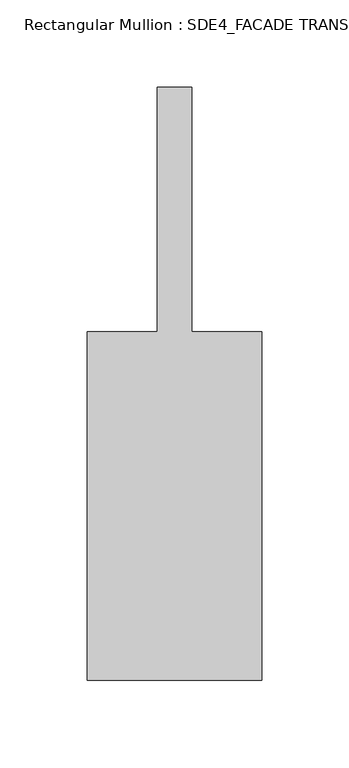
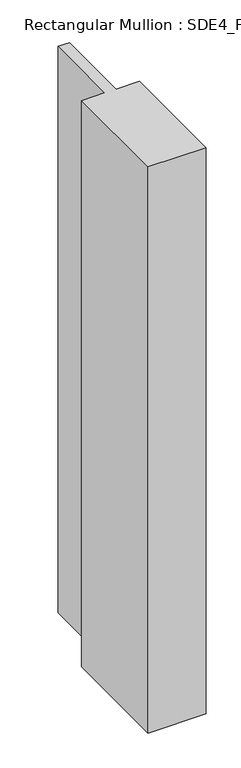
"""IFC4 building model written with IfcOpenShell, lengths in millimetres: member geometry, Rectangular Mullion : SDE4_FACADE TRANSOM TYPE 1."""

from ifc_helpers import new_model, si_unit, frame, origin, place, context, project, spatial, polyline, outline, extrude, source, transform, mapped, element, save


def rectangular_mullion_sde4_facade_transom_type_1_2f54afb5(model_context):
    return source(origin(), model_context, "Body", "SweptSolid", [
        extrude(outline(polyline([(50.0, -132.5), (-50.0, -132.5), (-50.0, 67.5), (-10.0, 67.5), (-10.0, 207.5), (10.0, 207.5), (10.0, 67.5), (50.0, 67.5), (50.0, -132.5)])), frame((0.0, 0.0, -1034.9624711), z_axis=(0.0, 0.0, 1.0), x_axis=(1.0, 0.0, 0.0)), (0.0, 0.0, 1.0), 1034.9624711),
    ])


if __name__ == "__main__":
    model = new_model("IFC4")
    model_context = context("Model", 3, world=origin())
    ifc_project = project(units=[si_unit("LENGTHUNIT", "METRE", prefix="MILLI")], contexts=[model_context])
    site = spatial("IfcSite", under=ifc_project)
    building = spatial("IfcBuilding", under=site)
    placement = place(None, origin())
    rectangular_mullion_sde4_facade_transom_type_1_shape = rectangular_mullion_sde4_facade_transom_type_1_2f54afb5(model_context)
    element("IfcMember", 1, ObjectType="Rectangular Mullion : SDE4_FACADE TRANSOM TYPE 1", at=placement, inside=building, context=model_context, shape_type="MappedRepresentation", body=[
        mapped(rectangular_mullion_sde4_facade_transom_type_1_shape, transform((0.0, 0.0, 0.0), x_axis=(1.0, 0.0, 0.0), y_axis=(0.0, 1.0, 0.0), z_axis=(0.0, 0.0, 1.0))),
    ])
    save(model, "model.ifc")

# Revit data of these elements
# Type "Rectangular Mullion : SDE4_FACADE TRANSOM TYPE 1"
#   built-in parameter 1007322 = 1.11549 (stored number, unit not read)
#   built-in parameter 1007321 = 0.164042 (stored number, unit not read)
#   built-in parameter 1007320 = 0.164042 (stored number, unit not read)
